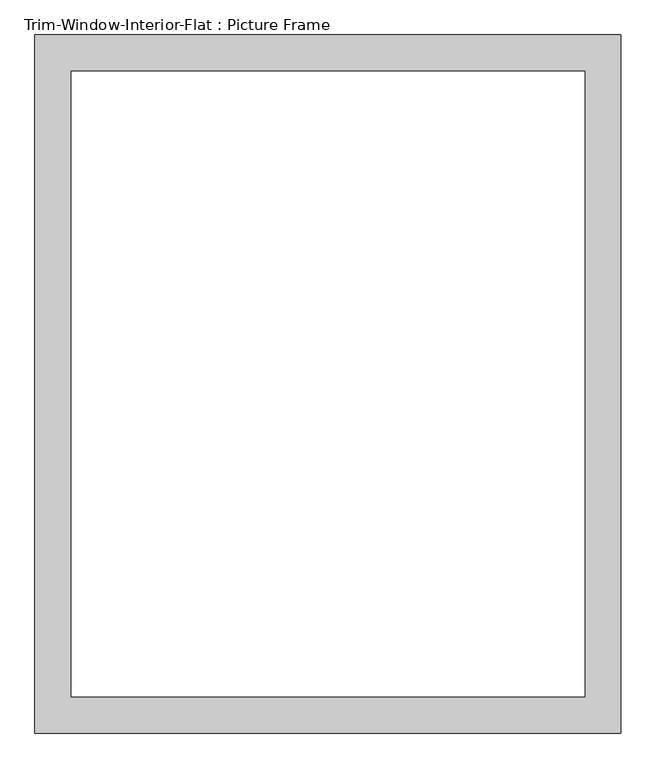
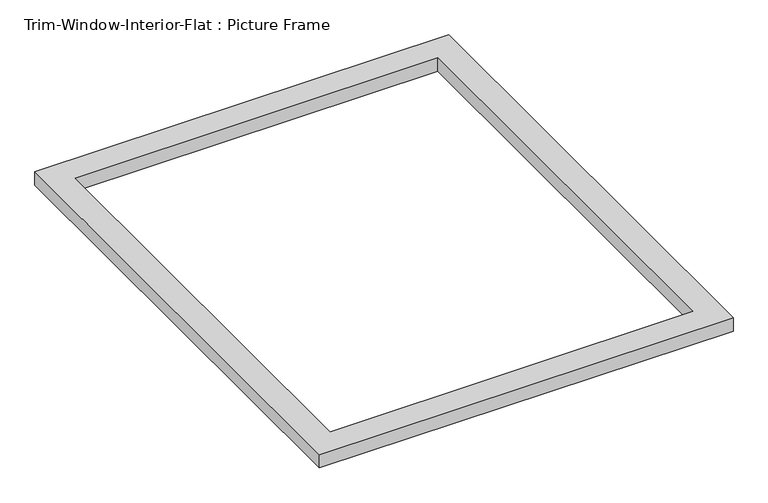
"""IFC4 building model written with IfcOpenShell, lengths in millimetres: proxy geometry, Trim-Window-Interior-Flat : Picture Frame."""

import ifcopenshell
import ifcopenshell.guid

model = None  # the IFC model being written
_history = None  # IfcOwnerHistory: only IFC2X3 demands one
_inside = {}  # id of a spatial element -> (the spatial element, [elements in it])
_under = {}  # id of a project, library or spatial element -> (it, [spatial elements below it])
_declared = {}  # id of a project -> (the project, [libraries it declares])
_typed = {}  # id of a type object -> (the type object, [elements of that type])
_made_of = {}  # id of a material, layer set ... -> (it, [elements and type objects made of it])


def new_model(schema):
    """Start an empty IFC model of exactly this schema.

    Asked for "IFC4X3", IfcOpenShell would pick the latest addendum, in which some entities
    have other attributes; the version numbers below select the first issue.
    IFC2X3 requires an IfcOwnerHistory on every rooted entity: one is made here for all.
    """
    global model, _history
    if schema == "IFC4X3":
        model = ifcopenshell.file(schema_version=(4, 3, 0, 0))
    else:
        model = ifcopenshell.file(schema=schema)
    _inside.clear()
    _under.clear()
    _declared.clear()
    _typed.clear()
    _made_of.clear()
    _history = None
    if model.schema == "IFC2X3":
        org = make("IfcOrganization", Name="unknown")
        user = make(
            "IfcPersonAndOrganization",
            ThePerson=make("IfcPerson", FamilyName="unknown"),
            TheOrganization=org,
        )
        app = make(
            "IfcApplication",
            ApplicationDeveloper=org,
            Version="unknown",
            ApplicationFullName="unknown",
            ApplicationIdentifier="unknown",
        )
        _history = make(
            "IfcOwnerHistory",
            OwningUser=user,
            OwningApplication=app,
            ChangeAction="ADDED",
            CreationDate=0,
        )
    return model


def make(cls, **values):
    """One entity of the class cls with the attributes given. An attribute that is None is left unset."""
    return model.create_entity(
        cls, **{name: value for name, value in values.items() if value is not None}
    )


def rooted(cls, **values):
    """An entity with a GlobalId (a new one), such as an element, a storey or a relation."""
    return make(cls, GlobalId=ifcopenshell.guid.new(), OwnerHistory=_history, **values)


def si_unit(unit_type, name, prefix=None):
    """IfcSIUnit, for example si_unit("LENGTHUNIT", "METRE", prefix="MILLI")."""
    return make("IfcSIUnit", UnitType=unit_type, Prefix=prefix, Name=name)


def assignment(units):
    """IfcUnitAssignment: the units of a project."""
    return None if units is None else make("IfcUnitAssignment", Units=units)


def point(xyz):
    """IfcCartesianPoint."""
    return None if xyz is None else make("IfcCartesianPoint", Coordinates=xyz)


def direction(xyz):
    """IfcDirection."""
    return None if xyz is None else make("IfcDirection", DirectionRatios=xyz)


def frame(location, z_axis=None, x_axis=None):
    """IfcAxis2Placement3D, a coordinate frame: its origin and axes. An axis left out is left unset."""
    return make(
        "IfcAxis2Placement3D",
        Location=point(location),
        Axis=direction(z_axis),
        RefDirection=direction(x_axis),
    )


def origin():
    """The frame at (0, 0, 0) with its axes left unset."""
    return frame((0.0, 0.0, 0.0))


def origin_with_axes():
    """The frame at (0, 0, 0) with the z axis (0, 0, 1) and the x axis (1, 0, 0) written out."""
    return frame((0.0, 0.0, 0.0), z_axis=(0.0, 0.0, 1.0), x_axis=(1.0, 0.0, 0.0))


def place(relative_to, where):
    """IfcLocalPlacement: puts the frame where relative to a parent placement (None: the world)."""
    return make(
        "IfcLocalPlacement", PlacementRelTo=relative_to, RelativePlacement=where
    )


def context(
    kind, dimensions, precision=None, world=None, true_north=None, identifier=None
):
    """IfcGeometricRepresentationContext, for example the 3D "Model" context."""
    return make(
        "IfcGeometricRepresentationContext",
        ContextIdentifier=identifier,
        ContextType=kind,
        CoordinateSpaceDimension=dimensions,
        Precision=precision,
        WorldCoordinateSystem=world,
        TrueNorth=true_north,
    )


def project(units=None, contexts=None):
    """IfcProject with its units and contexts."""
    return rooted(
        "IfcProject",
        Name="project",
        RepresentationContexts=contexts,
        UnitsInContext=assignment(units),
    )


def spatial(cls, under=None, at=None, **own):
    """A site, building, storey or space (cls), placed at a placement, below another one or the project."""
    s = rooted(cls, ObjectPlacement=at, **own)
    if under is not None:
        _under.setdefault(under.id(), (under, []))[1].append(s)
    return s


def polyline(points):
    """IfcPolyline through the points."""
    return make("IfcPolyline", Points=[point(p) for p in points])


def outline(outer, holes=None, kind="AREA"):
    """IfcArbitraryClosedProfileDef: a profile drawn as a closed curve; with holes, ...WithVoids."""
    if holes is None:
        return make("IfcArbitraryClosedProfileDef", ProfileType=kind, OuterCurve=outer)
    return make(
        "IfcArbitraryProfileDefWithVoids",
        ProfileType=kind,
        OuterCurve=outer,
        InnerCurves=holes,
    )


def extrude(swept, where, along, depth):
    """IfcExtrudedAreaSolid: the profile swept, set in the frame where, extruded along a direction by depth."""
    return make(
        "IfcExtrudedAreaSolid",
        SweptArea=swept,
        Position=where,
        ExtrudedDirection=direction(along),
        Depth=depth,
    )


def shape(context_of_items, identifier, shape_type, items):
    """IfcShapeRepresentation: the items that make up one representation, for example the "Body"."""
    return make(
        "IfcShapeRepresentation",
        ContextOfItems=context_of_items,
        RepresentationIdentifier=identifier,
        RepresentationType=shape_type,
        Items=items,
    )


def source(mapping_origin, context_of_items, identifier, shape_type, items):
    """IfcRepresentationMap: a shape defined once, which mapped items show again and again."""
    return make(
        "IfcRepresentationMap",
        MappingOrigin=mapping_origin,
        MappedRepresentation=shape(context_of_items, identifier, shape_type, items),
    )


def transform(
    local_origin,
    x_axis=None,
    y_axis=None,
    z_axis=None,
    scale=None,
    scale2=None,
    scale3=None,
    uniform=True,
):
    """IfcCartesianTransformationOperator3D, or its non-uniform kind. x_axis, y_axis, z_axis: its Axis1, 2, 3."""
    if uniform:
        return make(
            "IfcCartesianTransformationOperator3D",
            Axis1=direction(x_axis),
            Axis2=direction(y_axis),
            LocalOrigin=point(local_origin),
            Scale=scale,
            Axis3=direction(z_axis),
        )
    return make(
        "IfcCartesianTransformationOperator3DnonUniform",
        Axis1=direction(x_axis),
        Axis2=direction(y_axis),
        LocalOrigin=point(local_origin),
        Scale=scale,
        Axis3=direction(z_axis),
        Scale2=scale2,
        Scale3=scale3,
    )


def mapped(mapping_source, mapping_target):
    """IfcMappedItem: shows the shape of a source again, moved by a transform."""
    return make(
        "IfcMappedItem", MappingSource=mapping_source, MappingTarget=mapping_target
    )


def made_of(thing, what):
    """Note that an element or type object is made of a material, layer set ...; save() writes the relation."""
    if what is not None:
        _made_of.setdefault(what.id(), (what, []))[1].append(thing)
    return thing


def element(
    cls,
    number,
    at=None,
    inside=None,
    cuts=None,
    type_object=None,
    material=None,
    context=None,
    identifier="Body",
    shape_type=None,
    held_by="IfcProductDefinitionShape",
    body=None,
    shapes=None,
    **own,
):
    """One element of the class cls, such as IfcWall. Its Tag is "e" and its number.

    at: its placement. inside: the storey or other place that contains it. cuts: it is an
    opening in that element (IfcRelVoidsElement). A single representation is given by context,
    identifier, shape_type and body (its items); several are given by shapes. held_by: the class
    of the entity that holds the representations. save() writes the other relations.
    """
    e = rooted(cls, Tag="e%d" % number, ObjectPlacement=at, **own)
    if body is not None:
        shapes = [shape(context, identifier, shape_type, body)]
    if shapes is not None:
        e.Representation = make(held_by, Representations=shapes)
    if inside is not None:
        _inside.setdefault(inside.id(), (inside, []))[1].append(e)
    if cuts is not None:
        rooted(
            "IfcRelVoidsElement", RelatingBuildingElement=cuts, RelatedOpeningElement=e
        )
    if type_object is not None:
        _typed.setdefault(type_object.id(), (type_object, []))[1].append(e)
    return made_of(e, material)


def aggregate(whole, parts):
    """IfcRelAggregates: a whole, such as a stair, and the parts it consists of."""
    return rooted("IfcRelAggregates", RelatingObject=whole, RelatedObjects=parts)


def save(model, path):
    """Write the relations noted so far, then the file.

    IfcRelAggregates (storeys below a building ...), IfcRelContainedInSpatialStructure (elements
    in a storey), IfcRelDefinesByType, IfcRelAssociatesMaterial and IfcRelDeclares: one each for
    every whole, place, type object, material and project.
    """
    for whole, parts in _under.values():
        aggregate(whole, parts)
    for where, things in _inside.values():
        rooted(
            "IfcRelContainedInSpatialStructure",
            RelatedElements=things,
            RelatingStructure=where,
        )
    for kind, things in _typed.values():
        rooted("IfcRelDefinesByType", RelatedObjects=things, RelatingType=kind)
    for what, things in _made_of.values():
        rooted("IfcRelAssociatesMaterial", RelatedObjects=things, RelatingMaterial=what)
    for by, libraries in _declared.values():
        rooted("IfcRelDeclares", RelatingContext=by, RelatedDefinitions=libraries)
    model.write(path)


def trim_window_interior_flat_picture_frame_996979b4(model_context):
    return source(origin(), model_context, "Body", "SweptSolid", [
        extrude(outline(polyline([(463.55, 44.45), (463.55, -1060.45), (-463.55, -1060.45), (-463.55, 44.45), (463.55, 44.45)]), holes=[polyline([(406.4, -12.7), (-406.4, -12.7), (-406.4, -1003.3), (406.4, -1003.3), (406.4, -12.7)])]), origin_with_axes(), (0.0, 0.0, 1.0), 31.75),
    ])


if __name__ == "__main__":
    model = new_model("IFC4")
    model_context = context("Model", 3, world=origin())
    ifc_project = project(units=[si_unit("LENGTHUNIT", "METRE", prefix="MILLI")], contexts=[model_context])
    site = spatial("IfcSite", under=ifc_project)
    building = spatial("IfcBuilding", under=site)
    placement = place(None, origin())
    trim_window_interior_flat_picture_frame_shape = trim_window_interior_flat_picture_frame_996979b4(model_context)
    element("IfcBuildingElementProxy", 1, Name="Trim-Window-Interior-Flat : Picture Frame", ObjectType="Trim-Window-Interior-Flat : Picture Frame", at=placement, inside=building, context=model_context, shape_type="MappedRepresentation", body=[
        mapped(trim_window_interior_flat_picture_frame_shape, transform((0.0, 0.0, 0.0), x_axis=(1.0, 0.0, 0.0), y_axis=(0.0, 1.0, 0.0), z_axis=(0.0, 0.0, 1.0))),
    ])
    save(model, "model.ifc")

# Revit data of these elements
# Type "Trim-Window-Interior-Flat : Picture Frame"
#   Trim Thickness_Picture Frame = 0' - 1 1/4"
#   Trim Width = 0' - 2 1/4"
#   Trim Thickness_with Sill = 0' - 0 3/4"
#   Sill Thickness = 0' - 1 1/4"
#   Opening Width [instance default] = 2' - 0"
#   Opening Height [instance default] = 3' - 0"
#   Default Elevation = 4' - 0"
#   Sill = no
#   Picture Frame = yes
#   Trim Material [instance default] = none
# Element 1 (IfcBuildingElementProxy, "Trim-Window-Interior-Flat : Picture Frame")
#   Opening Width = 2' - 9"
#   Opening Height = 3' - 4"
#   Trim Material = 1X WOOD COMPOSITE TRIM
#   Materials on its faces: "1X WOOD COMPOSITE TRIM"
# Materials
#   "1X WOOD COMPOSITE TRIM": class "Generic", colour RGB 88 61 61, transparency 0, Cost = 0
